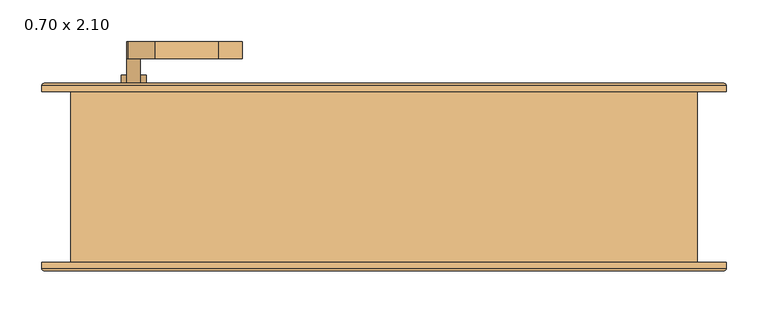
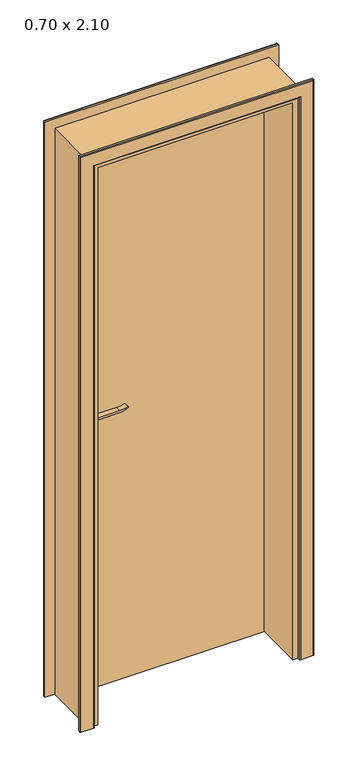
"""IFC4 building model written with IfcOpenShell, lengths in millimetres: door geometry, .CC_ND 300_PORTA SIMPLES DE ABRIR_COM EXTENSÃO : 0.70 x 2.10."""

from ifc_helpers import new_model, si_unit, point, frame, frame_2d, origin, origin_with_axes, place, context, project, spatial, polyline, circle_curve, ellipse_curve, trimmed, segment, composite_curve, outline, extrude, faceted_brep, source, transform, mapped, element, save
from ifc_brep_helpers import plane_surface, cylinder_surface, advanced_brep


def door_0_70_x_2_10_01854108(model_context):
    return source(origin(), model_context, "Body", "SolidModel", [
        extrude(outline(composite_curve([segment(trimmed(circle_curve(frame_2d((964.5, -300.0)), 15.0), [point((964.5, -285.0))], [point((964.5, -315.0))], False, "CARTESIAN"), True, "CONTINUOUS"), segment(trimmed(circle_curve(frame_2d((964.5, -300.0)), 15.0), [point((964.5, -315.0))], [point((964.5, -285.0))], False, "CARTESIAN"), True, "CONTINUOUS")], self_intersect=False)), frame((0.0, 127.9, 0.0), z_axis=(0.0, 1.0, 0.0), x_axis=(0.0, 0.0, 1.0)), (0.0, 0.0, 1.0), 10.0),
        extrude(outline(composite_curve([segment(trimmed(circle_curve(frame_2d((964.5, -300.0)), 15.0), [point((964.5, -285.0))], [point((964.5, -315.0))], False, "CARTESIAN"), True, "CONTINUOUS"), segment(trimmed(circle_curve(frame_2d((964.5, -300.0)), 15.0), [point((964.5, -315.0))], [point((964.5, -285.0))], False, "CARTESIAN"), True, "CONTINUOUS")], self_intersect=False)), frame((0.0, 67.9, 0.0), z_axis=(0.0, 1.0, 0.0), x_axis=(0.0, 0.0, 1.0)), (0.0, 0.0, 1.0), 10.0),
        extrude(outline(composite_curve([segment(trimmed(circle_curve(frame_2d((1024.5, -300.0)), 8.0), [point((1029.1523287, -306.5081363))], [point((1024.5, -292.0))], False, "CARTESIAN"), True, "CONTINUOUS"), segment(trimmed(circle_curve(frame_2d((1019.3738613, -274.6138099)), 18.1261387), [point((1024.5, -292.0))], [point((1037.5, -274.6138099))], True, "CARTESIAN"), True, "CONTINUOUS"), segment(polyline([(1037.5, -274.6138099), (1037.5, -198.3564091)]), True, "CONTINUOUS"), segment(trimmed(circle_curve(frame_2d((1096.7709207, -201.9396612)), 59.3791355), [point((1037.5, -198.3564091))], [point((1046.7135558, -170.0))], False, "CARTESIAN"), True, "CONTINUOUS"), segment(polyline([(1046.7135558, -170.0), (1049.5, -170.0)]), True, "CONTINUOUS"), segment(trimmed(circle_curve(frame_2d((1127.7850638, -198.4227909)), 83.2850902), [point((1049.5, -170.0))], [point((1044.5, -198.3564091))], True, "CARTESIAN"), True, "CONTINUOUS"), segment(polyline([(1044.5, -198.3564091), (1044.5, -274.6325667)]), True, "CONTINUOUS"), segment(trimmed(circle_curve(frame_2d((1007.2555521, -276.3324871)), 37.2832219), [point((1044.5, -274.6325667))], [point((1029.1523287, -306.5081363))], False, "CARTESIAN"), True, "CONTINUOUS")], self_intersect=False)), frame((0.0, 157.9, 0.0), z_axis=(0.0, 1.0, 0.0), x_axis=(0.0, 0.0, 1.0)), (0.0, 0.0, 1.0), 20.0),
        extrude(outline(composite_curve([segment(trimmed(circle_curve(frame_2d((1019.3738682, -274.6138122)), 18.1261318), [point((1024.4999903, -292.0))], [point((1037.5, -274.6138122))], True, "CARTESIAN"), True, "CONTINUOUS"), segment(polyline([(1037.5, -274.6138122), (1037.5, -198.3564091)]), True, "CONTINUOUS"), segment(trimmed(circle_curve(frame_2d((1096.7709207, -201.9396612)), 59.3791355), [point((1037.5, -198.3564091))], [point((1046.7135558, -170.0))], False, "CARTESIAN"), True, "CONTINUOUS"), segment(polyline([(1046.7135558, -170.0), (1049.5, -170.0)]), True, "CONTINUOUS"), segment(trimmed(circle_curve(frame_2d((1127.7850638, -198.4227909)), 83.2850902), [point((1049.5, -170.0))], [point((1044.5, -198.3564091))], True, "CARTESIAN"), True, "CONTINUOUS"), segment(polyline([(1044.5, -198.3564091), (1044.5, -274.6325667)]), True, "CONTINUOUS"), segment(trimmed(circle_curve(frame_2d((1007.2555521, -276.3324871)), 37.2832219), [point((1044.5, -274.6325667))], [point((1029.1523287, -306.5081363))], False, "CARTESIAN"), True, "CONTINUOUS"), segment(trimmed(circle_curve(frame_2d((1024.5, -300.0)), 8.0), [point((1029.1523287, -306.5081363))], [point((1024.4999903, -292.0))], False, "CARTESIAN"), True, "CONTINUOUS")], self_intersect=False)), frame((0.0, 27.9, 0.0), z_axis=(0.0, 1.0, 0.0), x_axis=(0.0, 0.0, 1.0)), (0.0, 0.0, 1.0), 20.0),
        extrude(outline(composite_curve([segment(trimmed(circle_curve(frame_2d((1024.5, -300.0)), 8.0), [point((1024.5, -292.0))], [point((1024.5, -308.0))], False, "CARTESIAN"), True, "CONTINUOUS"), segment(trimmed(circle_curve(frame_2d((1024.5, -300.0)), 8.0), [point((1024.5, -308.0))], [point((1024.5, -292.0))], False, "CARTESIAN"), True, "CONTINUOUS")], self_intersect=False)), frame((0.0, 127.9, 0.0), z_axis=(0.0, 1.0, 0.0), x_axis=(0.0, 0.0, 1.0)), (0.0, 0.0, 1.0), 30.0),
        extrude(outline(composite_curve([segment(trimmed(circle_curve(frame_2d((1024.5, -300.0)), 8.0), [point((1024.5, -292.0))], [point((1024.5, -308.0))], False, "CARTESIAN"), True, "CONTINUOUS"), segment(trimmed(circle_curve(frame_2d((1024.5, -300.0)), 8.0), [point((1024.5, -308.0))], [point((1024.5, -292.0))], False, "CARTESIAN"), True, "CONTINUOUS")], self_intersect=False)), frame((0.0, 47.9, 0.0), z_axis=(0.0, 1.0, 0.0), x_axis=(0.0, 0.0, 1.0)), (0.0, 0.0, 1.0), 30.0),
        extrude(outline(composite_curve([segment(trimmed(circle_curve(frame_2d((954.5, -300.0)), 25.0), [point((954.5, -325.0))], [point((954.5, -275.0))], False, "CARTESIAN"), True, "CONTINUOUS"), segment(polyline([(954.5, -275.0), (1024.5, -275.0)]), True, "CONTINUOUS"), segment(trimmed(circle_curve(frame_2d((1024.5, -300.0)), 25.0), [point((1024.5, -275.0))], [point((1024.5, -325.0))], False, "CARTESIAN"), True, "CONTINUOUS"), segment(polyline([(1024.5, -325.0), (954.5, -325.0)]), True, "CONTINUOUS")], self_intersect=False)), frame((0.0, 117.9, 0.0), z_axis=(0.0, 1.0, 0.0), x_axis=(0.0, 0.0, 1.0)), (0.0, 0.0, 1.0), 10.0),
        extrude(outline(composite_curve([segment(trimmed(circle_curve(frame_2d((954.5, -300.0)), 25.0), [point((954.5, -325.0))], [point((954.5, -275.0))], False, "CARTESIAN"), True, "CONTINUOUS"), segment(polyline([(954.5, -275.0), (1024.5, -275.0)]), True, "CONTINUOUS"), segment(trimmed(circle_curve(frame_2d((1024.5, -300.0)), 25.0), [point((1024.5, -275.0))], [point((1024.5, -325.0))], False, "CARTESIAN"), True, "CONTINUOUS"), segment(polyline([(1024.5, -325.0), (954.5, -325.0)]), True, "CONTINUOUS")], self_intersect=False)), frame((0.0, 77.9, 0.0), z_axis=(0.0, 1.0, 0.0), x_axis=(0.0, 0.0, 1.0)), (0.0, 0.0, 1.0), 10.0),
        advanced_brep(
        [(-410.0, 117.9, 0.0), (-410.0, 124.9, 0.0), (-407.0, 127.9, 0.0), (-363.0, 127.9, 0.0), (-360.0, 124.9, 0.0), (-360.0, 117.9, 0.0), (-360.0, 117.9, 2085.0), (360.0, 117.9, 2085.0), (360.0, 117.9, 0.0), (410.0, 117.9, 0.0), (410.0, 117.9, 2135.0), (-410.0, 117.9, 2135.0), (-360.0, 124.9, 2085.0), (-363.0, 127.9, 2088.0), (-407.0, 127.9, 2132.0), (407.0, 127.9, 2132.0), (407.0, 127.9, 0.0), (363.0, 127.9, 0.0), (363.0, 127.9, 2088.0), (-410.0, 124.9, 2135.0), (410.0, 124.9, 0.0), (410.0, 124.9, 2135.0), (360.0, 124.9, 0.0), (360.0, 124.9, 2085.0)],
        [
            (0, 1),
            (1, 2, circle_curve(frame((-407.0, 124.9, 0.0), z_axis=(0.0, 0.0, -1.0), x_axis=(1.0, 0.0, 0.0)), 3.0)),
            (2, 3),
            (3, 4, circle_curve(frame((-363.0, 124.9, 0.0), z_axis=(0.0, 0.0, -1.0), x_axis=(1.0, 0.0, 0.0)), 3.0)),
            (4, 5),
            (5, 0),
            (5, 6),
            (6, 7),
            (7, 8),
            (8, 9),
            (9, 10),
            (10, 11),
            (11, 0),
            (4, 12),
            (12, 6),
            (3, 13),
            (13, 12, ellipse_curve(frame((-363.0, 124.9, 2088.0), z_axis=(-0.7071067811865475, 0.0, -0.7071067811865475), x_axis=(0.7071067811865474, 0.0, -0.7071067811865476)), 4.2426407, 3.0)),
            (2, 14),
            (14, 15),
            (15, 16),
            (16, 17),
            (17, 18),
            (18, 13),
            (1, 19),
            (19, 14, ellipse_curve(frame((-407.0, 124.9, 2132.0), z_axis=(-0.7071067811865475, 0.0, -0.7071067811865475), x_axis=(0.7071067811865474, 0.0, -0.7071067811865476)), 4.2426407, 3.0)),
            (11, 19),
            (9, 20),
            (20, 21),
            (21, 10),
            (8, 22),
            (22, 17, circle_curve(frame((363.0, 124.9, 0.0), z_axis=(0.0, 0.0, -1.0), x_axis=(-1.0, 0.0, 0.0)), 3.0)),
            (16, 20, circle_curve(frame((407.0, 124.9, 0.0), z_axis=(0.0, 0.0, -1.0), x_axis=(-1.0, 0.0, 0.0)), 3.0)),
            (23, 22),
            (7, 23),
            (23, 18, ellipse_curve(frame((363.0, 124.9, 2088.0), z_axis=(0.7071067811865475, 0.0, -0.7071067811865475), x_axis=(0.7071067811865474, 0.0, 0.7071067811865476)), 4.2426407, 3.0)),
            (15, 21, ellipse_curve(frame((407.0, 124.9, 2132.0), z_axis=(0.7071067811865475, 0.0, -0.7071067811865475), x_axis=(0.7071067811865474, 0.0, 0.7071067811865476)), 4.2426407, 3.0)),
            (12, 23),
            (21, 19),
        ],
        [
            plane_surface(frame((-360.0, 117.9, 0.0), z_axis=(0.0, 0.0, -1.0), x_axis=(0.0, -1.0, 0.0))),
            plane_surface(frame((-410.0, 117.9, 0.0), z_axis=(0.0, -1.0, 0.0), x_axis=(0.0, 0.0, 1.0))),
            plane_surface(frame((-360.0, 117.9, 0.0), z_axis=(1.0, 0.0, 0.0), x_axis=(0.0, 0.0, 1.0))),
            cylinder_surface(frame((-363.0, 124.9, 0.0), z_axis=(0.0, 0.0, -1.0), x_axis=(1.0, 0.0, 0.0)), 3.0),
            plane_surface(frame((-363.0, 127.9, 0.0), z_axis=(0.0, 1.0, 0.0), x_axis=(0.0, 0.0, 1.0))),
            cylinder_surface(frame((-407.0, 124.9, 0.0), z_axis=(0.0, 0.0, -1.0), x_axis=(1.0, 0.0, 0.0)), 3.0),
            plane_surface(frame((-410.0, 124.9, 0.0), z_axis=(-1.0, 0.0, 0.0), x_axis=(0.0, 0.0, 1.0))),
            plane_surface(frame((410.0, 124.9, 2135.0), z_axis=(1.0, 0.0, 0.0), x_axis=(0.0, 0.0, -1.0))),
            plane_surface(frame((360.0, 117.9, 0.0), z_axis=(0.0, 0.0, -1.0), x_axis=(0.0, -1.0, 0.0))),
            plane_surface(frame((360.0, 117.9, 2085.0), z_axis=(-1.0, 0.0, 0.0), x_axis=(0.0, 0.0, -1.0))),
            cylinder_surface(frame((363.0, 124.9, 2085.0), z_axis=(0.0, 0.0, 1.0), x_axis=(-1.0, 0.0, 0.0)), 3.0),
            cylinder_surface(frame((407.0, 124.9, 2085.0), z_axis=(0.0, 0.0, 1.0), x_axis=(-1.0, 0.0, 0.0)), 3.0),
            plane_surface(frame((-360.0, 117.9, 2085.0), z_axis=(0.0, 0.0, -1.0), x_axis=(1.0, 0.0, 0.0))),
            plane_surface(frame((-410.0, 124.9, 2135.0), z_axis=(0.0, 0.0, 1.0), x_axis=(1.0, 0.0, 0.0))),
            cylinder_surface(frame((-360.0, 124.9, 2088.0), z_axis=(-1.0, 0.0, 0.0), x_axis=(0.0, 0.0, -1.0)), 3.0),
            cylinder_surface(frame((-360.0, 124.9, 2132.0), z_axis=(-1.0, 0.0, 0.0), x_axis=(0.0, 0.0, -1.0)), 3.0),
        ],
        [
            (0, [[1, 2, 3, 4, 5, 6]]),
            (1, [[7, 8, 9, 10, 11, 12, 13, -6]]),
            (2, [[14, 15, -7, -5]]),
            (3, [[16, 17, -14, -4]]),
            (4, [[18, 19, 20, 21, 22, 23, -16, -3]]),
            (5, [[24, 25, -18, -2]]),
            (6, [[-13, 26, -24, -1]]),
            (7, [[-11, 27, 28, 29]]),
            (8, [[-10, 30, 31, -21, 32, -27]]),
            (9, [[33, -30, -9, 34]]),
            (10, [[-22, -31, -33, 35]]),
            (11, [[-28, -32, -20, 36]]),
            (12, [[37, -34, -8, -15]]),
            (13, [[-12, -29, 38, -26]]),
            (14, [[-23, -35, -37, -17]]),
            (15, [[-38, -36, -19, -25]]),
        ],
    ),
        advanced_brep(
        [(410.0, -86.9, 0.0), (410.0, -93.9342217, 0.0), (407.0342217, -96.9, 0.0), (362.9842717, -96.9, 0.0), (360.0, -93.9157283, 0.0), (360.0, -86.9, 0.0), (360.0, -86.9, 2085.0), (-360.0, -86.9, 2085.0), (-360.0, -86.9, 0.0), (-410.0, -86.9, 0.0), (-410.0, -86.9, 2135.0), (410.0, -86.9, 2135.0), (360.0, -93.9157283, 2085.0), (362.9842717, -96.9, 2087.9842717), (407.0342217, -96.9, 2132.0342217), (-407.0342217, -96.9, 2132.0342217), (-407.0342217, -96.9, 0.0), (-362.9842717, -96.9, 0.0), (-362.9842717, -96.9, 2087.9842717), (410.0, -93.9342217, 2135.0), (-410.0, -93.9342217, 0.0), (-410.0, -93.9342217, 2135.0), (-360.0, -93.9157283, 0.0), (-360.0, -93.9157283, 2085.0)],
        [
            (0, 1),
            (1, 2, circle_curve(frame((407.0342217, -93.9342217, 0.0), z_axis=(0.0, 0.0, -1.0), x_axis=(1.0, 0.0, 0.0)), 2.9657783)),
            (2, 3),
            (3, 4, circle_curve(frame((362.9842717, -93.9157283, 0.0), z_axis=(0.0, 0.0, -1.0), x_axis=(1.0, 0.0, 0.0)), 2.9842717)),
            (4, 5),
            (5, 0),
            (5, 6),
            (6, 7),
            (7, 8),
            (8, 9),
            (9, 10),
            (10, 11),
            (11, 0),
            (4, 12),
            (12, 6),
            (3, 13),
            (13, 12, ellipse_curve(frame((362.9842717, -93.9157283, 2087.9842717), z_axis=(0.7071067811865475, 0.0, -0.7071067811865475), x_axis=(-0.7071067811865474, 0.0, -0.7071067811865476)), 4.2203975, 2.9842717)),
            (2, 14),
            (14, 15),
            (15, 16),
            (16, 17),
            (17, 18),
            (18, 13),
            (1, 19),
            (19, 14, ellipse_curve(frame((407.0342217, -93.9342217, 2132.0342217), z_axis=(0.7071067811865475, 0.0, -0.7071067811865475), x_axis=(-0.7071067811865474, 0.0, -0.7071067811865476)), 4.1942438, 2.9657783)),
            (11, 19),
            (9, 20),
            (20, 21),
            (21, 10),
            (8, 22),
            (22, 17, circle_curve(frame((-362.9842717, -93.9157283, 0.0), z_axis=(0.0, 0.0, -1.0), x_axis=(-1.0, 0.0, 0.0)), 2.9842717)),
            (16, 20, circle_curve(frame((-407.0342217, -93.9342217, 0.0), z_axis=(0.0, 0.0, -1.0), x_axis=(-1.0, 0.0, 0.0)), 2.9657783)),
            (23, 22),
            (7, 23),
            (23, 18, ellipse_curve(frame((-362.9842717, -93.9157283, 2087.9842717), z_axis=(-0.7071067811865475, 0.0, -0.7071067811865475), x_axis=(-0.7071067811865474, 0.0, 0.7071067811865476)), 4.2203975, 2.9842717)),
            (15, 21, ellipse_curve(frame((-407.0342217, -93.9342217, 2132.0342217), z_axis=(-0.7071067811865475, 0.0, -0.7071067811865475), x_axis=(-0.7071067811865474, 0.0, 0.7071067811865476)), 4.1942438, 2.9657783)),
            (12, 23),
            (21, 19),
        ],
        [
            plane_surface(frame((360.0, -86.9, 0.0), z_axis=(0.0, 0.0, -1.0), x_axis=(0.0, -1.0, 0.0))),
            plane_surface(frame((410.0, -86.9, 0.0), z_axis=(0.0, 1.0, 0.0), x_axis=(0.0, 0.0, 1.0))),
            plane_surface(frame((360.0, -86.9, 0.0), z_axis=(-1.0, 0.0, 0.0), x_axis=(0.0, 0.0, 1.0))),
            cylinder_surface(frame((362.9842717, -93.9157283, 0.0), z_axis=(0.0, 0.0, -1.0), x_axis=(1.0, 0.0, 0.0)), 2.9842717),
            plane_surface(frame((362.9842717, -96.9, 0.0), z_axis=(0.0, -1.0, 0.0), x_axis=(0.0, 0.0, 1.0))),
            cylinder_surface(frame((407.0342217, -93.9342217, 0.0), z_axis=(0.0, 0.0, -1.0), x_axis=(1.0, 0.0, 0.0)), 2.9657783),
            plane_surface(frame((410.0, -93.9342217, 0.0), z_axis=(1.0, 0.0, 0.0), x_axis=(0.0, 0.0, 1.0))),
            plane_surface(frame((-410.0, -93.9342217, 2135.0), z_axis=(-1.0, 0.0, 0.0), x_axis=(0.0, 0.0, -1.0))),
            plane_surface(frame((-360.0, -86.9, 0.0), z_axis=(0.0, 0.0, -1.0), x_axis=(0.0, -1.0, 0.0))),
            plane_surface(frame((-360.0, -86.9, 2085.0), z_axis=(1.0, 0.0, 0.0), x_axis=(0.0, 0.0, -1.0))),
            cylinder_surface(frame((-362.9842717, -93.9157283, 2085.0), z_axis=(0.0, 0.0, 1.0), x_axis=(-1.0, 0.0, 0.0)), 2.9842717),
            cylinder_surface(frame((-407.0342217, -93.9342217, 2085.0), z_axis=(0.0, 0.0, 1.0), x_axis=(-1.0, 0.0, 0.0)), 2.9657783),
            plane_surface(frame((360.0, -86.9, 2085.0), z_axis=(0.0, 0.0, -1.0), x_axis=(-1.0, 0.0, 0.0))),
            plane_surface(frame((410.0, -93.9342217, 2135.0), z_axis=(0.0, 0.0, 1.0), x_axis=(-1.0, 0.0, 0.0))),
            cylinder_surface(frame((360.0, -93.9157283, 2087.9842717), z_axis=(1.0, 0.0, 0.0), x_axis=(0.0, 0.0, 1.0)), 2.9842717),
            cylinder_surface(frame((360.0, -93.9342217, 2132.0342217), z_axis=(1.0, 0.0, 0.0), x_axis=(0.0, 0.0, 1.0)), 2.9657783),
        ],
        [
            (0, [[1, 2, 3, 4, 5, 6]]),
            (1, [[7, 8, 9, 10, 11, 12, 13, -6]]),
            (2, [[14, 15, -7, -5]]),
            (3, [[16, 17, -14, -4]]),
            (4, [[18, 19, 20, 21, 22, 23, -16, -3]]),
            (5, [[24, 25, -18, -2]]),
            (6, [[-13, 26, -24, -1]]),
            (7, [[-11, 27, 28, 29]]),
            (8, [[-10, 30, 31, -21, 32, -27]]),
            (9, [[33, -30, -9, 34]]),
            (10, [[-22, -31, -33, 35]]),
            (11, [[-28, -32, -20, 36]]),
            (12, [[37, -34, -8, -15]]),
            (13, [[-12, -29, 38, -26]]),
            (14, [[-23, -35, -37, -17]]),
            (15, [[-38, -36, -19, -25]]),
        ],
    ),
        faceted_brep([(342.0, -86.9, 0.0), (342.0, 87.9, 0.0), (350.0, 87.9, 0.0), (350.0, 117.9, 0.0), (375.0, 117.9, 0.0), (375.0, -86.9, 0.0), (375.0, -86.9, 2100.0), (-375.0, -86.9, 2100.0), (-375.0, -86.9, 0.0), (-342.0, -86.9, 0.0), (-342.0, -86.9, 2067.0), (342.0, -86.9, 2067.0), (375.0, 117.9, 2100.0), (350.0, 117.9, 2075.0), (-350.0, 117.9, 2075.0), (-350.0, 117.9, 0.0), (-375.0, 117.9, 0.0), (-375.0, 117.9, 2100.0), (350.0, 87.9, 2075.0), (342.0, 87.9, 2067.0), (-342.0, 87.9, 2067.0), (-342.0, 87.9, 0.0), (-350.0, 87.9, 0.0), (-350.0, 87.9, 2075.0)], [[[0, 1, 2, 3, 4, 5]], [[5, 6, 7, 8, 9, 10, 11, 0]], [[4, 12, 6, 5]], [[3, 13, 14, 15, 16, 17, 12, 4]], [[2, 18, 13, 3]], [[1, 19, 20, 21, 22, 23, 18, 2]], [[0, 11, 19, 1]], [[10, 9, 21, 20]], [[9, 8, 16, 15, 22, 21]], [[17, 16, 8, 7]], [[23, 22, 15, 14]], [[12, 17, 7, 6]], [[18, 23, 14, 13]], [[11, 10, 20, 19]]]),
        extrude(outline(polyline([(-350.0, 87.9), (-350.0, 117.9), (350.0, 117.9), (350.0, 87.9), (-350.0, 87.9)])), origin_with_axes(), (0.0, 0.0, 1.0), 2075.0),
    ])


if __name__ == "__main__":
    model = new_model("IFC4")
    model_context = context("Model", 3, world=origin())
    ifc_project = project(units=[si_unit("LENGTHUNIT", "METRE", prefix="MILLI")], contexts=[model_context])
    site = spatial("IfcSite", under=ifc_project)
    building = spatial("IfcBuilding", under=site)
    placement = place(None, origin())
    door_0_70_x_2_10_shape = door_0_70_x_2_10_01854108(model_context)
    element("IfcDoor", 1, ObjectType=".CC_ND 300_PORTA SIMPLES DE ABRIR_COM EXTENSÃO : 0.70 x 2.10", at=placement, inside=building, context=model_context, shape_type="MappedRepresentation", body=[
        mapped(door_0_70_x_2_10_shape, transform((0.0, 0.0, 0.0), x_axis=(1.0, 0.0, 0.0), y_axis=(0.0, 1.0, 0.0), z_axis=(0.0, 0.0, 1.0))),
    ])
    save(model, "model.ifc")

# Revit data of these elements
# Project information
#   Design Option = "Main Model"
#   Project Status = "Status do projeto"
#   Project Address = "RUA SÉRGIO DIAS, LOTE 30, QUADRA G, MONTE MINEIRO/MG"
#   Project Name = "RESIDÊNCIA - ROBERTA VENDRAMINI"
#   Project Number = "034/2017"
#   Zona = "ZER - 01"
#   CA Mín = "0.2"
#   CA Básico = "1"
#   CA Máx = "2"
#   TO Máx = "50"
#   Gabarito Máx = "10"
#   TP Mín = "15"
#   Área Total do Terreno = "620.00 m²"
#   Multifamiliar - Vagas Veículos/Pavto = "0"
#   Multifamiliar - Vagas Bicicletas/Pavto = "0"
#   Multifamiliar - % Vagas PNMR = "0"
#   Multifamiliar - % Vagas Motos = "0"
#   Outros - Área p/ 1 Veículo = "0.00 m²"
#   Outros - Área p/ 1 Bicicleta = "0.00 m²"
#   Outros - Área p/ 1 Utilitário = "0.00 m²"
#   Outros - % Vagas PNMR = "0"
#   Outros - % Vagas Motos = "0"
# Type ".CC_ND 300_PORTA SIMPLES DE ABRIR_COM EXTENSÃO : 0.70 x 2.10"
#   Type Mark = "155"
#   Rough Width = 0.75 m
#   Espessura moldura externa = 0.01 m
#   Espessura moldura interna = 0.01 m
#   Largura moldura = 0.05 m
#   Extensão acabamento exterior [instance default] = 0.00 m
#   Extensão acabamento interior [instance default] = 0.00 m
#   Espessura batente = 0.025 m
#   Thickness = 0.03 m
#   Altura batente = 2.085 m
#   Aux Arco [instance default] = 0.70 m
#   Rough Height = 2.125 m
#   Height = 2.10 m
#   Width = 0.70 m
#   Moldura interna [instance default] = yes
#   Moldura externa [instance default] = yes
#   Porta = .MADEIRA COM PINTURA ESMALTE BRANCO ACETINADO
#   Moldura = .MADEIRA COM PINTURA ESMALTE BRANCO ACETINADO
#   Maçaneta = .ALUMÍNIO
#   Batente = .MADEIRA COM PINTURA ESMALTE BRANCO ACETINADO
#   Function = (empty or 0)
#   Wall Closure = (empty or 0)
# Element 1 (IfcDoor, ".CC_ND 300_PORTA SIMPLES DE ABRIR_COM EXTENSÃO : 0.70 x 2.10")
#   Extensão acabamento interior = 0.031 m
#   Aux Arco = 0.731 m
#   Materials on its faces: ".MADEIRA COM PINTURA ESMALTE BRANCO ACETINADO", ".ALUMÍNIO"
# Materials
#   ".MADEIRA COM PINTURA ESMALTE BRANCO ACETINADO": class ".CC_MADEIRAS", colour RGB 240 240 240, transparency 0, Description = "Madeira com pintura esmalte branco acetinado.", Cost = 0
#   ".ALUMÍNIO": class "CC_METAIS", colour RGB 244 244 244, transparency 0, Description = "Material alumínio", Cost = 0
